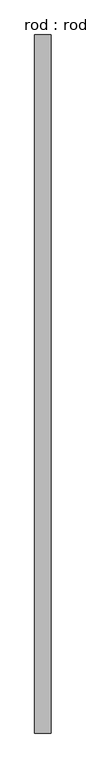
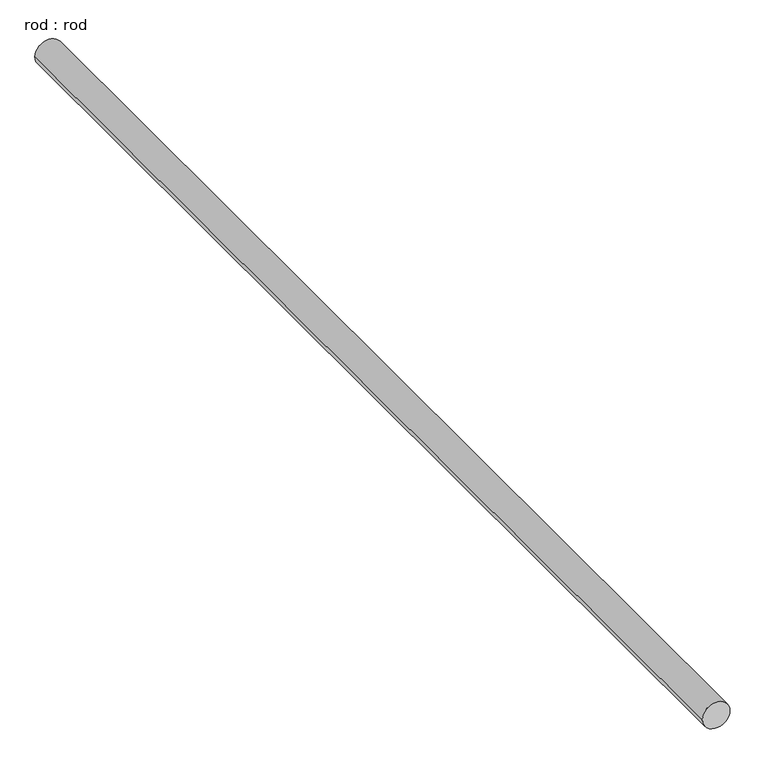
"""IFC4 building model written with IfcOpenShell, lengths in millimetres: proxy geometry, rod : rod."""

from ifc_helpers import new_model, si_unit, point, frame, frame_2d, origin, place, context, project, spatial, circle_curve, trimmed, segment, composite_curve, outline, extrude, source, transform, mapped, element, save


def rod_rod_07d07971(model_context):
    return source(origin(), model_context, "Body", "SweptSolid", [
        extrude(outline(composite_curve([segment(trimmed(circle_curve(frame_2d((0.0108462, 0.0)), 200.0), [point((0.0108462, 200.0))], [point((0.0108462, -200.0))], False, "CARTESIAN"), True, "CONTINUOUS"), segment(trimmed(circle_curve(frame_2d((0.0108462, 0.0)), 200.0), [point((0.0108462, -200.0))], [point((0.0108462, 200.0))], False, "CARTESIAN"), True, "CONTINUOUS")], self_intersect=False)), frame((0.0, -4331.3785275, 0.0), z_axis=(0.0, 1.0, 0.0), x_axis=(0.0, 0.0, 1.0)), (0.0, 0.0, 1.0), 16848.2142857),
    ])


if __name__ == "__main__":
    model = new_model("IFC4")
    model_context = context("Model", 3, world=origin())
    ifc_project = project(units=[si_unit("LENGTHUNIT", "METRE", prefix="MILLI")], contexts=[model_context])
    site = spatial("IfcSite", under=ifc_project)
    building = spatial("IfcBuilding", under=site)
    placement = place(None, origin())
    rod_rod_shape = rod_rod_07d07971(model_context)
    element("IfcBuildingElementProxy", 1, Name="rod : rod", ObjectType="rod : rod", at=placement, inside=building, context=model_context, shape_type="MappedRepresentation", body=[
        mapped(rod_rod_shape, transform((0.0, 0.0, 0.0), x_axis=(1.0, 0.0, 0.0), y_axis=(0.0, 1.0, 0.0), z_axis=(0.0, 0.0, 1.0))),
    ])
    save(model, "model.ifc")

# Revit data of these elements
# Type "rod : rod"
#   Default Elevation = 0
